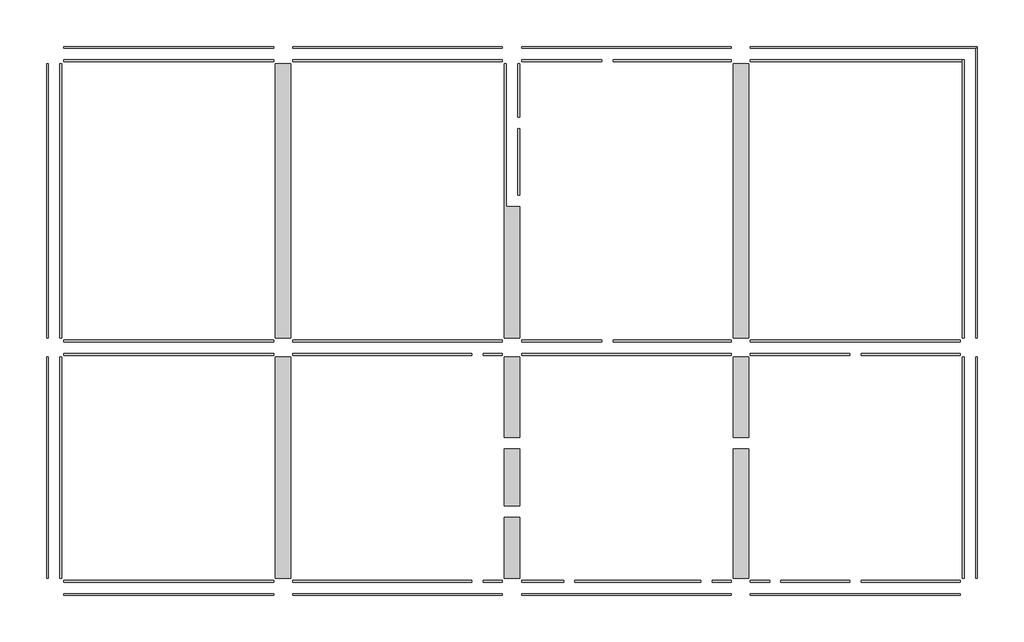
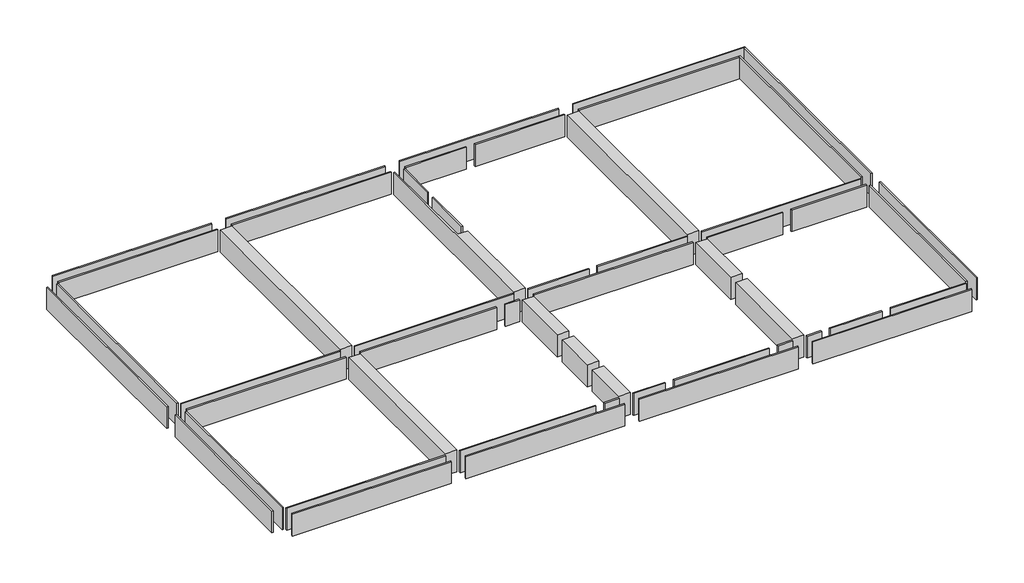
# One storey: 22 beams.
"""IFC4 building model written with IfcOpenShell, lengths in millimetres."""

from ifc_helpers import new_model, si_unit, frame, origin, place, context, project, spatial, polyline, outline, extrude, faceted_brep, element, save

model = new_model("IFC4")

# Units and contexts
model_context = context("Model", 3, world=origin())
ifc_project = project(units=[si_unit("LENGTHUNIT", "METRE", prefix="MILLI")], contexts=[model_context])

# Site, building, storey
site = spatial("IfcSite", under=ifc_project)
building = spatial("IfcBuilding", under=site)
storey = spatial("IfcBuildingStorey", under=building, Name="2nd FL GL+6,200", Elevation=6000.0)

# Beams
placement = place(None, origin())
element("IfcBeam", 1, ObjectType="콘크리트-직사각형 보 : 400 x 800mm", at=placement, inside=storey, context=model_context, shape_type="Brep", body=[
    faceted_brep([(-445.7273237, 9285.9763125, 6000.0), (-445.7273237, 9235.9763125, 6000.0), (5104.2726763, 9235.9763125, 6000.0), (5104.2726763, 9285.9763125, 6000.0), (-445.7273237, 9235.9763125, 5200.0), (-445.7273237, 9285.9763125, 5200.0), (5104.2726763, 9285.9763125, 5200.0), (5104.2726763, 9235.9763125, 5200.0)], [[[0, 1, 2, 3]], [[4, 1, 0, 5]], [[5, 0, 3, 6]], [[4, 5, 6, 7]], [[1, 4, 7, 2]], [[3, 2, 7, 6]]]),
    faceted_brep([(-445.7273237, 9635.9763125, 5200.0), (-445.7273237, 9635.9763125, 6000.0), (5504.2726763, 9635.9763125, 6000.0), (5504.2726763, 9635.9763125, 5200.0), (5504.2726763, 9585.9763125, 5200.0), (5454.2726763, 9585.9763125, 5200.0), (-445.7273237, 9585.9763125, 5200.0), (-445.7273237, 9585.9763125, 6000.0), (5504.2726763, 9585.9763125, 6000.0), (5454.2726763, 9585.9763125, 6000.0)], [[[0, 1, 2, 3]], [[4, 5, 6, 0, 3]], [[7, 6, 5, 4, 8, 9]], [[1, 0, 6, 7]], [[3, 2, 8, 4]], [[1, 7, 9, 8, 2]]]),
])
element("IfcBeam", 2, ObjectType="콘크리트-직사각형 보 : 400 x 800mm", at=placement, inside=storey, context=model_context, shape_type="SweptSolid", body=[
    extrude(outline(polyline([(-6445.7273237, 9235.9763125), (-6445.7273237, 9285.9763125), (-4345.7273237, 9285.9763125), (-4345.7273237, 9235.9763125), (-6445.7273237, 9235.9763125)])), frame((0.0, 0.0, 5200.0), z_axis=(0.0, 0.0, 1.0), x_axis=(1.0, 0.0, 0.0)), (0.0, 0.0, 1.0), 800.0),
    extrude(outline(polyline([(-6445.7273237, 9635.9763125), (-945.7273237, 9635.9763125), (-945.7273237, 9585.9763125), (-6445.7273237, 9585.9763125), (-6445.7273237, 9635.9763125)])), frame((0.0, 0.0, 5200.0), z_axis=(0.0, 0.0, 1.0), x_axis=(1.0, 0.0, 0.0)), (0.0, 0.0, 1.0), 800.0),
    extrude(outline(polyline([(-945.7273237, 9285.9763125), (-945.7273237, 9235.9763125), (-4045.7273237, 9235.9763125), (-4045.7273237, 9285.9763125), (-945.7273237, 9285.9763125)])), frame((0.0, 0.0, 5200.0), z_axis=(0.0, 0.0, 1.0), x_axis=(1.0, 0.0, 0.0)), (0.0, 0.0, 1.0), 800.0),
])
element("IfcBeam", 3, ObjectType="콘크리트-직사각형 보 : 400 x 800mm", at=placement, inside=storey, context=model_context, shape_type="SweptSolid", body=[
    extrude(outline(polyline([(-12445.7273237, 9235.9763125), (-12445.7273237, 9285.9763125), (-6945.7273237, 9285.9763125), (-6945.7273237, 9235.9763125), (-12445.7273237, 9235.9763125)])), frame((0.0, 0.0, 5200.0), z_axis=(0.0, 0.0, 1.0), x_axis=(1.0, 0.0, 0.0)), (0.0, 0.0, 1.0), 800.0),
    extrude(outline(polyline([(-12445.7273237, 9585.9763125), (-12445.7273237, 9635.9763125), (-6945.7273237, 9635.9763125), (-6945.7273237, 9585.9763125), (-12445.7273237, 9585.9763125)])), frame((0.0, 0.0, 5200.0), z_axis=(0.0, 0.0, 1.0), x_axis=(1.0, 0.0, 0.0)), (0.0, 0.0, 1.0), 800.0),
])
element("IfcBeam", 4, ObjectType="콘크리트-직사각형 보 : 400 x 800mm", at=placement, inside=storey, context=model_context, shape_type="SweptSolid", body=[
    extrude(outline(polyline([(-12945.7273237, 9235.9763125), (-18445.7273237, 9235.9763125), (-18445.7273237, 9285.9763125), (-12945.7273237, 9285.9763125), (-12945.7273237, 9235.9763125)])), frame((0.0, 0.0, 5200.0), z_axis=(0.0, 0.0, 1.0), x_axis=(1.0, 0.0, 0.0)), (0.0, 0.0, 1.0), 800.0),
    extrude(outline(polyline([(-18445.7273237, 9635.9763125), (-12945.7273237, 9635.9763125), (-12945.7273237, 9585.9763125), (-18445.7273237, 9585.9763125), (-18445.7273237, 9635.9763125)])), frame((0.0, 0.0, 5200.0), z_axis=(0.0, 0.0, 1.0), x_axis=(1.0, 0.0, 0.0)), (0.0, 0.0, 1.0), 800.0),
])
element("IfcBeam", 5, ObjectType="콘크리트-직사각형 보 : 400 x 800mm", at=placement, inside=storey, context=model_context, shape_type="SweptSolid", body=[
    extrude(outline(polyline([(-18895.7273237, -4314.0236875), (-18895.7273237, 1485.9763125), (-18845.7273237, 1485.9763125), (-18845.7273237, -4314.0236875), (-18895.7273237, -4314.0236875)])), frame((0.0, 0.0, 5200.0), z_axis=(0.0, 0.0, 1.0), x_axis=(1.0, 0.0, 0.0)), (0.0, 0.0, 1.0), 800.0),
    extrude(outline(polyline([(-18495.7273237, 1485.9763125), (-18495.7273237, -4314.0236875), (-18545.7273237, -4314.0236875), (-18545.7273237, 1485.9763125), (-18495.7273237, 1485.9763125)])), frame((0.0, 0.0, 5200.0), z_axis=(0.0, 0.0, 1.0), x_axis=(1.0, 0.0, 0.0)), (0.0, 0.0, 1.0), 800.0),
])
element("IfcBeam", 6, ObjectType="콘크리트-직사각형 보 : 400 x 800mm", at=placement, inside=storey, context=model_context, shape_type="SweptSolid", body=[
    extrude(outline(polyline([(-18895.7273237, 1985.9763125), (-18895.7273237, 9185.9763125), (-18845.7273237, 9185.9763125), (-18845.7273237, 1985.9763125), (-18895.7273237, 1985.9763125)])), frame((0.0, 0.0, 5200.0), z_axis=(0.0, 0.0, 1.0), x_axis=(1.0, 0.0, 0.0)), (0.0, 0.0, 1.0), 800.0),
    extrude(outline(polyline([(-18495.7273237, 9185.9763125), (-18495.7273237, 1985.9763125), (-18545.7273237, 1985.9763125), (-18545.7273237, 9185.9763125), (-18495.7273237, 9185.9763125)])), frame((0.0, 0.0, 5200.0), z_axis=(0.0, 0.0, 1.0), x_axis=(1.0, 0.0, 0.0)), (0.0, 0.0, 1.0), 800.0),
])
element("IfcBeam", 7, ObjectType="콘크리트-직사각형 보 : 400 x 800mm", at=placement, inside=storey, context=model_context, shape_type="SweptSolid", body=[
    extrude(outline(polyline([(-12895.7273237, 1485.9763125), (-12495.7273237, 1485.9763125), (-12495.7273237, -4314.0236875), (-12895.7273237, -4314.0236875), (-12895.7273237, 1485.9763125)])), frame((0.0, 0.0, 5200.0), z_axis=(0.0, 0.0, 1.0), x_axis=(1.0, 0.0, 0.0)), (0.0, 0.0, 1.0), 800.0),
])
element("IfcBeam", 8, ObjectType="콘크리트-직사각형 보 : 400 x 800mm", at=placement, inside=storey, context=model_context, shape_type="SweptSolid", body=[
    extrude(outline(polyline([(-12895.7273237, 9185.9763125), (-12495.7273237, 9185.9763125), (-12495.7273237, 1985.9763125), (-12895.7273237, 1985.9763125), (-12895.7273237, 9185.9763125)])), frame((0.0, 0.0, 5200.0), z_axis=(0.0, 0.0, 1.0), x_axis=(1.0, 0.0, 0.0)), (0.0, 0.0, 1.0), 800.0),
])
element("IfcBeam", 9, ObjectType="콘크리트-직사각형 보 : 400 x 800mm", at=placement, inside=storey, context=model_context, shape_type="SweptSolid", body=[
    extrude(outline(polyline([(-6895.7273237, 1485.9763125), (-6495.7273237, 1485.9763125), (-6495.7273237, -614.0236875), (-6895.7273237, -614.0236875), (-6895.7273237, 1485.9763125)])), frame((0.0, 0.0, 5200.0), z_axis=(0.0, 0.0, 1.0), x_axis=(1.0, 0.0, 0.0)), (0.0, 0.0, 1.0), 800.0),
    extrude(outline(polyline([(-6495.7273237, -4314.0236875), (-6895.7273237, -4314.0236875), (-6895.7273237, -2714.0236875), (-6495.7273237, -2714.0236875), (-6495.7273237, -4314.0236875)])), frame((0.0, 0.0, 5200.0), z_axis=(0.0, 0.0, 1.0), x_axis=(1.0, 0.0, 0.0)), (0.0, 0.0, 1.0), 800.0),
    extrude(outline(polyline([(-6895.7273237, -914.0236875), (-6495.7273237, -914.0236875), (-6495.7273237, -2414.0236875), (-6895.7273237, -2414.0236875), (-6895.7273237, -914.0236875)])), frame((0.0, 0.0, 5200.0), z_axis=(0.0, 0.0, 1.0), x_axis=(1.0, 0.0, 0.0)), (0.0, 0.0, 1.0), 800.0),
])
element("IfcBeam", 10, ObjectType="콘크리트-직사각형 보 : 400 x 800mm", at=placement, inside=storey, context=model_context, shape_type="Brep", body=[
    faceted_brep([(-6895.7273237, 1985.9763125, 6000.0), (-6495.7273237, 1985.9763125, 6000.0), (-6495.7273237, 5435.9763125, 6000.0), (-6845.7273237, 5435.9763125, 6000.0), (-6845.7273237, 5735.9763125, 6000.0), (-6845.7273237, 9185.9763125, 6000.0), (-6895.7273237, 9185.9763125, 6000.0), (-6495.7273237, 1985.9763125, 5200.0), (-6495.7273237, 5435.9763125, 5200.0), (-6895.7273237, 9185.9763125, 5200.0), (-6895.7273237, 1985.9763125, 5200.0), (-6845.7273237, 9185.9763125, 5200.0), (-6845.7273237, 5435.9763125, 5200.0)], [[[0, 1, 2, 3, 4, 5, 6]], [[1, 7, 8, 2]], [[6, 9, 10, 0]], [[9, 6, 5, 11]], [[1, 0, 10, 7]], [[3, 2, 8, 12]], [[3, 12, 11, 5, 4]], [[7, 10, 9, 11, 12, 8]]]),
    faceted_brep([(-6495.7273237, 5735.9763125, 5200.0), (-6545.7273237, 5735.9763125, 5200.0), (-6545.7273237, 7485.9763125, 5200.0), (-6495.7273237, 7485.9763125, 5200.0), (-6495.7273237, 5735.9763125, 6000.0), (-6545.7273237, 5735.9763125, 6000.0), (-6545.7273237, 7485.9763125, 6000.0), (-6495.7273237, 7485.9763125, 6000.0)], [[[0, 1, 2, 3]], [[0, 4, 5, 1]], [[1, 5, 6, 2]], [[3, 2, 6, 7]], [[4, 0, 3, 7]], [[5, 4, 7, 6]]]),
    faceted_brep([(-6495.7273237, 9185.9763125, 5200.0), (-6495.7273237, 9185.9763125, 6000.0), (-6495.7273237, 7785.9763125, 6000.0), (-6495.7273237, 7785.9763125, 5200.0), (-6545.7273237, 9185.9763125, 6000.0), (-6545.7273237, 7785.9763125, 6000.0), (-6545.7273237, 9185.9763125, 5200.0), (-6545.7273237, 7785.9763125, 5200.0)], [[[0, 1, 2, 3]], [[1, 4, 5, 2]], [[1, 0, 6, 4]], [[7, 3, 2, 5]], [[6, 0, 3, 7]], [[4, 6, 7, 5]]]),
])
element("IfcBeam", 11, ObjectType="콘크리트-직사각형 보 : 400 x 800mm", at=placement, inside=storey, context=model_context, shape_type="SweptSolid", body=[
    extrude(outline(polyline([(-895.7273237, 1485.9763125), (-495.7273237, 1485.9763125), (-495.7273237, -614.0236875), (-895.7273237, -614.0236875), (-895.7273237, 1485.9763125)])), frame((0.0, 0.0, 5200.0), z_axis=(0.0, 0.0, 1.0), x_axis=(1.0, 0.0, 0.0)), (0.0, 0.0, 1.0), 800.0),
    extrude(outline(polyline([(-495.7273237, -4314.0236875), (-895.7273237, -4314.0236875), (-895.7273237, -914.0236875), (-495.7273237, -914.0236875), (-495.7273237, -4314.0236875)])), frame((0.0, 0.0, 5200.0), z_axis=(0.0, 0.0, 1.0), x_axis=(1.0, 0.0, 0.0)), (0.0, 0.0, 1.0), 800.0),
])
element("IfcBeam", 12, ObjectType="콘크리트-직사각형 보 : 400 x 800mm", at=placement, inside=storey, context=model_context, shape_type="SweptSolid", body=[
    extrude(outline(polyline([(-895.7273237, 9185.9763125), (-495.7273237, 9185.9763125), (-495.7273237, 1985.9763125), (-895.7273237, 1985.9763125), (-895.7273237, 9185.9763125)])), frame((0.0, 0.0, 5200.0), z_axis=(0.0, 0.0, 1.0), x_axis=(1.0, 0.0, 0.0)), (0.0, 0.0, 1.0), 800.0),
])
element("IfcBeam", 13, ObjectType="콘크리트-직사각형 보 : 400 x 800mm", at=placement, inside=storey, context=model_context, shape_type="SweptSolid", body=[
    extrude(outline(polyline([(5104.2726763, 1485.9763125), (5154.2726763, 1485.9763125), (5154.2726763, -4314.0236875), (5104.2726763, -4314.0236875), (5104.2726763, 1485.9763125)])), frame((0.0, 0.0, 5200.0), z_axis=(0.0, 0.0, 1.0), x_axis=(1.0, 0.0, 0.0)), (0.0, 0.0, 1.0), 800.0),
    extrude(outline(polyline([(5454.2726763, 1485.9763125), (5504.2726763, 1485.9763125), (5504.2726763, -4314.0236875), (5454.2726763, -4314.0236875), (5454.2726763, 1485.9763125)])), frame((0.0, 0.0, 5200.0), z_axis=(0.0, 0.0, 1.0), x_axis=(1.0, 0.0, 0.0)), (0.0, 0.0, 1.0), 800.0),
])
element("IfcBeam", 14, ObjectType="콘크리트-직사각형 보 : 400 x 800mm", at=placement, inside=storey, context=model_context, shape_type="Brep", body=[
    faceted_brep([(5154.2726763, 9285.9763125, 6000.0), (5104.2726763, 9285.9763125, 6000.0), (5104.2726763, 9235.9763125, 6000.0), (5104.2726763, 1985.9763125, 6000.0), (5154.2726763, 1985.9763125, 6000.0), (5104.2726763, 9285.9763125, 5200.0), (5104.2726763, 9235.9763125, 5200.0), (5104.2726763, 1985.9763125, 5200.0), (5154.2726763, 9285.9763125, 5200.0), (5154.2726763, 1985.9763125, 5200.0)], [[[0, 1, 2, 3, 4]], [[1, 5, 6, 7, 3, 2]], [[5, 1, 0, 8]], [[8, 0, 4, 9]], [[5, 8, 9, 7, 6]], [[4, 3, 7, 9]]]),
    faceted_brep([(5504.2726763, 9585.9763125, 5200.0), (5504.2726763, 9585.9763125, 6000.0), (5504.2726763, 1985.9763125, 6000.0), (5504.2726763, 1985.9763125, 5200.0), (5454.2726763, 9585.9763125, 5200.0), (5454.2726763, 1985.9763125, 5200.0), (5454.2726763, 9585.9763125, 6000.0), (5454.2726763, 1985.9763125, 6000.0), (5454.2726763, 9285.9763125, 6000.0)], [[[0, 1, 2, 3]], [[4, 0, 3, 5]], [[1, 0, 4, 6]], [[6, 4, 5, 7, 8]], [[1, 6, 8, 7, 2]], [[3, 2, 7, 5]]]),
])
element("IfcBeam", 15, ObjectType="콘크리트-직사각형 보 : 400 x 800mm", at=placement, inside=storey, context=model_context, shape_type="SweptSolid", body=[
    extrude(outline(polyline([(-445.7273237, 1535.9763125), (-445.7273237, 1585.9763125), (2154.2726763, 1585.9763125), (2154.2726763, 1535.9763125), (-445.7273237, 1535.9763125)])), frame((0.0, 0.0, 5200.0), z_axis=(0.0, 0.0, 1.0), x_axis=(1.0, 0.0, 0.0)), (0.0, 0.0, 1.0), 800.0),
    extrude(outline(polyline([(-445.7273237, 1935.9763125), (5054.2726763, 1935.9763125), (5054.2726763, 1885.9763125), (-445.7273237, 1885.9763125), (-445.7273237, 1935.9763125)])), frame((0.0, 0.0, 5200.0), z_axis=(0.0, 0.0, 1.0), x_axis=(1.0, 0.0, 0.0)), (0.0, 0.0, 1.0), 800.0),
    extrude(outline(polyline([(5054.2726763, 1585.9763125), (5054.2726763, 1535.9763125), (2454.2726763, 1535.9763125), (2454.2726763, 1585.9763125), (5054.2726763, 1585.9763125)])), frame((0.0, 0.0, 5200.0), z_axis=(0.0, 0.0, 1.0), x_axis=(1.0, 0.0, 0.0)), (0.0, 0.0, 1.0), 800.0),
])
element("IfcBeam", 16, ObjectType="콘크리트-직사각형 보 : 400 x 800mm", at=placement, inside=storey, context=model_context, shape_type="SweptSolid", body=[
    extrude(outline(polyline([(-945.7273237, 1535.9763125), (-6445.7273237, 1535.9763125), (-6445.7273237, 1585.9763125), (-945.7273237, 1585.9763125), (-945.7273237, 1535.9763125)])), frame((0.0, 0.0, 5200.0), z_axis=(0.0, 0.0, 1.0), x_axis=(1.0, 0.0, 0.0)), (0.0, 0.0, 1.0), 800.0),
    extrude(outline(polyline([(-4045.7273237, 1885.9763125), (-4045.7273237, 1935.9763125), (-945.7273237, 1935.9763125), (-945.7273237, 1885.9763125), (-4045.7273237, 1885.9763125)])), frame((0.0, 0.0, 5200.0), z_axis=(0.0, 0.0, 1.0), x_axis=(1.0, 0.0, 0.0)), (0.0, 0.0, 1.0), 800.0),
    extrude(outline(polyline([(-4345.7273237, 1935.9763125), (-4345.7273237, 1885.9763125), (-6445.7273237, 1885.9763125), (-6445.7273237, 1935.9763125), (-4345.7273237, 1935.9763125)])), frame((0.0, 0.0, 5200.0), z_axis=(0.0, 0.0, 1.0), x_axis=(1.0, 0.0, 0.0)), (0.0, 0.0, 1.0), 800.0),
])
element("IfcBeam", 17, ObjectType="콘크리트-직사각형 보 : 400 x 800mm", at=placement, inside=storey, context=model_context, shape_type="SweptSolid", body=[
    extrude(outline(polyline([(-12445.7273237, 1535.9763125), (-12445.7273237, 1585.9763125), (-7745.7273237, 1585.9763125), (-7745.7273237, 1535.9763125), (-12445.7273237, 1535.9763125)])), frame((0.0, 0.0, 5200.0), z_axis=(0.0, 0.0, 1.0), x_axis=(1.0, 0.0, 0.0)), (0.0, 0.0, 1.0), 800.0),
    extrude(outline(polyline([(-12445.7273237, 1885.9763125), (-12445.7273237, 1935.9763125), (-6945.7273237, 1935.9763125), (-6945.7273237, 1885.9763125), (-12445.7273237, 1885.9763125)])), frame((0.0, 0.0, 5200.0), z_axis=(0.0, 0.0, 1.0), x_axis=(1.0, 0.0, 0.0)), (0.0, 0.0, 1.0), 800.0),
    extrude(outline(polyline([(-6945.7273237, 1585.9763125), (-6945.7273237, 1535.9763125), (-7445.7273237, 1535.9763125), (-7445.7273237, 1585.9763125), (-6945.7273237, 1585.9763125)])), frame((0.0, 0.0, 5200.0), z_axis=(0.0, 0.0, 1.0), x_axis=(1.0, 0.0, 0.0)), (0.0, 0.0, 1.0), 800.0),
])
element("IfcBeam", 18, ObjectType="콘크리트-직사각형 보 : 400 x 800mm", at=placement, inside=storey, context=model_context, shape_type="SweptSolid", body=[
    extrude(outline(polyline([(-12945.7273237, 1535.9763125), (-18445.7273237, 1535.9763125), (-18445.7273237, 1585.9763125), (-12945.7273237, 1585.9763125), (-12945.7273237, 1535.9763125)])), frame((0.0, 0.0, 5200.0), z_axis=(0.0, 0.0, 1.0), x_axis=(1.0, 0.0, 0.0)), (0.0, 0.0, 1.0), 800.0),
    extrude(outline(polyline([(-18445.7273237, 1935.9763125), (-12945.7273237, 1935.9763125), (-12945.7273237, 1885.9763125), (-18445.7273237, 1885.9763125), (-18445.7273237, 1935.9763125)])), frame((0.0, 0.0, 5200.0), z_axis=(0.0, 0.0, 1.0), x_axis=(1.0, 0.0, 0.0)), (0.0, 0.0, 1.0), 800.0),
])
element("IfcBeam", 19, ObjectType="콘크리트-직사각형 보 : 400 x 800mm", at=placement, inside=storey, context=model_context, shape_type="SweptSolid", body=[
    extrude(outline(polyline([(5054.2726763, -4764.0236875), (-445.7273237, -4764.0236875), (-445.7273237, -4714.0236875), (5054.2726763, -4714.0236875), (5054.2726763, -4764.0236875)])), frame((0.0, 0.0, 5200.0), z_axis=(0.0, 0.0, 1.0), x_axis=(1.0, 0.0, 0.0)), (0.0, 0.0, 1.0), 800.0),
    extrude(outline(polyline([(-445.7273237, -4414.0236875), (-445.7273237, -4364.0236875), (54.2726763, -4364.0236875), (54.2726763, -4414.0236875), (-445.7273237, -4414.0236875)])), frame((0.0, 0.0, 5200.0), z_axis=(0.0, 0.0, 1.0), x_axis=(1.0, 0.0, 0.0)), (0.0, 0.0, 1.0), 800.0),
    extrude(outline(polyline([(5054.2726763, -4364.0236875), (5054.2726763, -4414.0236875), (2454.2726763, -4414.0236875), (2454.2726763, -4364.0236875), (5054.2726763, -4364.0236875)])), frame((0.0, 0.0, 5200.0), z_axis=(0.0, 0.0, 1.0), x_axis=(1.0, 0.0, 0.0)), (0.0, 0.0, 1.0), 800.0),
    extrude(outline(polyline([(2154.2726763, -4364.0236875), (2154.2726763, -4414.0236875), (354.2726763, -4414.0236875), (354.2726763, -4364.0236875), (2154.2726763, -4364.0236875)])), frame((0.0, 0.0, 5200.0), z_axis=(0.0, 0.0, 1.0), x_axis=(1.0, 0.0, 0.0)), (0.0, 0.0, 1.0), 800.0),
])
element("IfcBeam", 20, ObjectType="콘크리트-직사각형 보 : 400 x 800mm", at=placement, inside=storey, context=model_context, shape_type="SweptSolid", body=[
    extrude(outline(polyline([(-945.7273237, -4764.0236875), (-6445.7273237, -4764.0236875), (-6445.7273237, -4714.0236875), (-945.7273237, -4714.0236875), (-945.7273237, -4764.0236875)])), frame((0.0, 0.0, 5200.0), z_axis=(0.0, 0.0, 1.0), x_axis=(1.0, 0.0, 0.0)), (0.0, 0.0, 1.0), 800.0),
    extrude(outline(polyline([(-945.7273237, -4364.0236875), (-945.7273237, -4414.0236875), (-1445.7273237, -4414.0236875), (-1445.7273237, -4364.0236875), (-945.7273237, -4364.0236875)])), frame((0.0, 0.0, 5200.0), z_axis=(0.0, 0.0, 1.0), x_axis=(1.0, 0.0, 0.0)), (0.0, 0.0, 1.0), 800.0),
    extrude(outline(polyline([(-6445.7273237, -4414.0236875), (-6445.7273237, -4364.0236875), (-5345.7273237, -4364.0236875), (-5345.7273237, -4414.0236875), (-6445.7273237, -4414.0236875)])), frame((0.0, 0.0, 5200.0), z_axis=(0.0, 0.0, 1.0), x_axis=(1.0, 0.0, 0.0)), (0.0, 0.0, 1.0), 800.0),
    extrude(outline(polyline([(-5045.7273237, -4414.0236875), (-5045.7273237, -4364.0236875), (-1745.7273237, -4364.0236875), (-1745.7273237, -4414.0236875), (-5045.7273237, -4414.0236875)])), frame((0.0, 0.0, 5200.0), z_axis=(0.0, 0.0, 1.0), x_axis=(1.0, 0.0, 0.0)), (0.0, 0.0, 1.0), 800.0),
])
element("IfcBeam", 21, ObjectType="콘크리트-직사각형 보 : 400 x 800mm", at=placement, inside=storey, context=model_context, shape_type="SweptSolid", body=[
    extrude(outline(polyline([(-6945.7273237, -4764.0236875), (-12445.7273237, -4764.0236875), (-12445.7273237, -4714.0236875), (-6945.7273237, -4714.0236875), (-6945.7273237, -4764.0236875)])), frame((0.0, 0.0, 5200.0), z_axis=(0.0, 0.0, 1.0), x_axis=(1.0, 0.0, 0.0)), (0.0, 0.0, 1.0), 800.0),
    extrude(outline(polyline([(-6945.7273237, -4364.0236875), (-6945.7273237, -4414.0236875), (-7445.7273237, -4414.0236875), (-7445.7273237, -4364.0236875), (-6945.7273237, -4364.0236875)])), frame((0.0, 0.0, 5200.0), z_axis=(0.0, 0.0, 1.0), x_axis=(1.0, 0.0, 0.0)), (0.0, 0.0, 1.0), 800.0),
    extrude(outline(polyline([(-12445.7273237, -4414.0236875), (-12445.7273237, -4364.0236875), (-7745.7273237, -4364.0236875), (-7745.7273237, -4414.0236875), (-12445.7273237, -4414.0236875)])), frame((0.0, 0.0, 5200.0), z_axis=(0.0, 0.0, 1.0), x_axis=(1.0, 0.0, 0.0)), (0.0, 0.0, 1.0), 800.0),
])
element("IfcBeam", 22, ObjectType="콘크리트-직사각형 보 : 400 x 800mm", at=placement, inside=storey, context=model_context, shape_type="SweptSolid", body=[
    extrude(outline(polyline([(-12945.7273237, -4714.0236875), (-12945.7273237, -4764.0236875), (-18445.7273237, -4764.0236875), (-18445.7273237, -4714.0236875), (-12945.7273237, -4714.0236875)])), frame((0.0, 0.0, 5200.0), z_axis=(0.0, 0.0, 1.0), x_axis=(1.0, 0.0, 0.0)), (0.0, 0.0, 1.0), 800.0),
    extrude(outline(polyline([(-12945.7273237, -4364.0236875), (-12945.7273237, -4414.0236875), (-18445.7273237, -4414.0236875), (-18445.7273237, -4364.0236875), (-12945.7273237, -4364.0236875)])), frame((0.0, 0.0, 5200.0), z_axis=(0.0, 0.0, 1.0), x_axis=(1.0, 0.0, 0.0)), (0.0, 0.0, 1.0), 800.0),
])

save(model, "model.ifc")

# Revit data of these elements
# Type "콘크리트-직사각형 보 : 400 x 800mm"
#   Length [instance default] = 1524 mm
#   b = 400 mm
#   h = 800 mm
#   Structural Material [instance default] = 콘크리트, 현장타설 회색
#   Assembly Code = ""
# Elements 1, 2, 3, 4, 5, 6, 7, 8, 9, 10, 11, 12, 13, 14, 15, 16, 17, 18, 19, 20, 21, 22 (IfcBeam, "콘크리트-직사각형 보 : 400 x 800mm")
#   Structural Material = 콘크리트, 현장타설 회색
#   Phase Created = 신축
#   Materials on its faces: "콘크리트, 현장타설 회색"
# Materials
#   "콘크리트, 현장타설 회색": class "콘크리트", colour RGB 192 192 192, transparency 0, Description = "현장타설 콘크리트", Cost = 0
